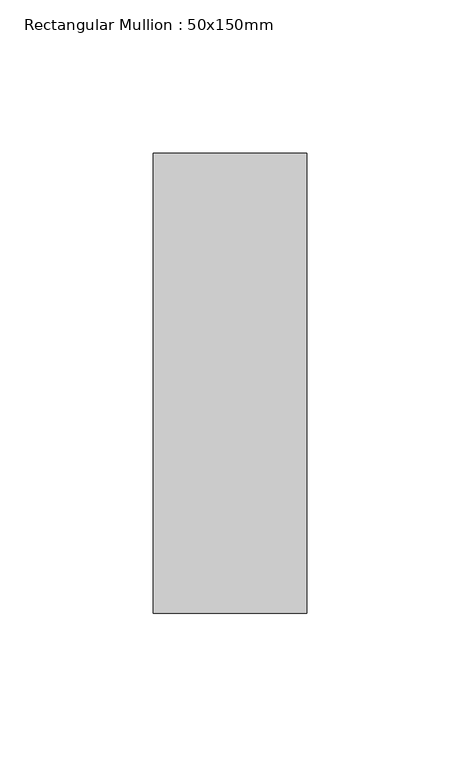
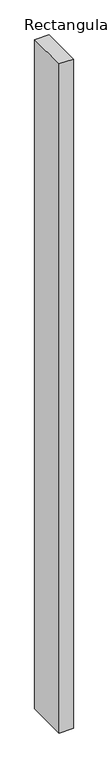
"""IFC4 building model written with IfcOpenShell, lengths in millimetres: member geometry, Rectangular Mullion : 50x150mm."""

from ifc_helpers import new_model, si_unit, frame, origin, place, context, project, spatial, polyline, outline, extrude, source, transform, mapped, element, save


def rectangular_mullion_50x150mm_4c3b9bdb(model_context):
    return source(origin(), model_context, "Body", "SweptSolid", [
        extrude(outline(polyline([(0.0, 75.0), (0.0, -75.0), (-50.0, -75.0), (-50.0, 75.0), (0.0, 75.0)])), frame((0.0, 0.0, -2500.0), z_axis=(0.0, 0.0, 1.0), x_axis=(1.0, 0.0, 0.0)), (0.0, 0.0, 1.0), 2500.0),
    ])


if __name__ == "__main__":
    model = new_model("IFC4")
    model_context = context("Model", 3, world=origin())
    ifc_project = project(units=[si_unit("LENGTHUNIT", "METRE", prefix="MILLI")], contexts=[model_context])
    site = spatial("IfcSite", under=ifc_project)
    building = spatial("IfcBuilding", under=site)
    placement = place(None, origin())
    rectangular_mullion_50x150mm_shape = rectangular_mullion_50x150mm_4c3b9bdb(model_context)
    element("IfcMember", 1, ObjectType="Rectangular Mullion : 50x150mm", at=placement, inside=building, context=model_context, shape_type="MappedRepresentation", body=[
        mapped(rectangular_mullion_50x150mm_shape, transform((0.0, 0.0, 0.0), x_axis=(1.0, 0.0, 0.0), y_axis=(0.0, 1.0, 0.0), z_axis=(0.0, 0.0, 1.0))),
    ])
    save(model, "model.ifc")

# Revit data of these elements
# Type "Rectangular Mullion : 50x150mm"
#   Keynote = "H11"
#   built-in parameter 1007304 = 0.492126 (stored number, unit not read)
#   built-in parameter 1007301 = 0.082021 (stored number, unit not read)
#   built-in parameter 1007300 = 0.082021 (stored number, unit not read)
# Element 1 (IfcMember, "Rectangular Mullion : 50x150mm")
#   Materials on its faces: "Aluminium"
# Materials
#   "Aluminium": class "Metal", colour RGB 247 247 247, transparency 0, Description = "Aluminium 6061", Cost = 0
